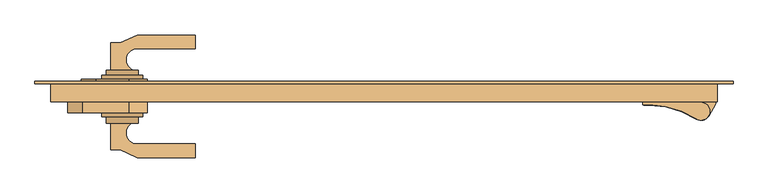
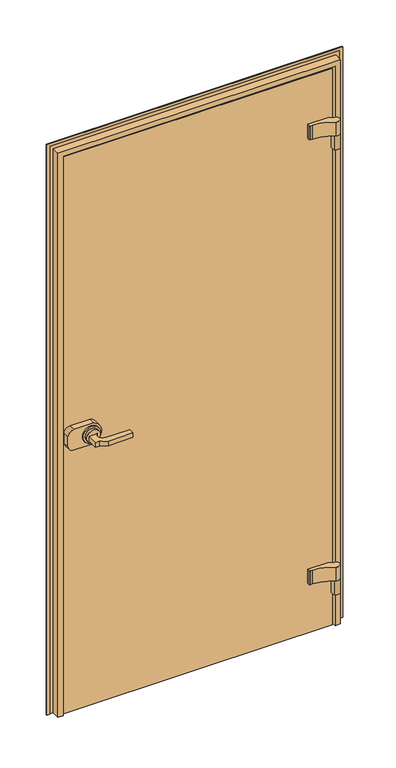
"""IFC4 building model written with IfcOpenShell, lengths in millimetres: door geometry, Doors_Doors_Faraone_Anta : Doors_Doors_Faraone_Anta."""

from ifc_helpers import new_model, si_unit, point, frame, frame_2d, origin, place, context, project, spatial, polyline, circle_curve, trimmed, segment, composite_curve, outline, extrude, faceted_brep, source, transform, mapped, element, save


def door_472ffe8c(model_context):
    return source(origin(), model_context, "Body", "SolidModel", [
        extrude(outline(polyline([(376.5509112, 11.599726), (446.250386, 11.599726), (446.250386, 1.8997991), (376.5509112, 1.8997991), (376.5509112, 11.599726)])), frame((0.0, 0.0, 1799.0000277), z_axis=(0.0, 0.0, 1.0), x_axis=(1.0, 0.0, 0.0)), (0.0, 0.0, 1.0), 50.0),
        extrude(outline(composite_curve([segment(polyline([(376.5509112, -17.600054), (376.5509112, -8.1001256), (446.5503838, -8.1001256), (446.5503838, -9.6001143), (466.1896331, -16.9560894)]), True, "CONTINUOUS"), segment(trimmed(circle_curve(frame_2d((461.5502708, -29.0999673)), 12.9999021), [point((466.1896331, -16.9560894))], [point((454.7624862, -40.1870515))], False, "CARTESIAN"), True, "CONTINUOUS"), segment(trimmed(circle_curve(frame_2d((385.1363002, -147.5843675)), 127.9921454), [point((454.7624862, -40.1870515))], [point((386.5508359, -19.6000389))], True, "CARTESIAN"), True, "CONTINUOUS"), segment(polyline([(386.5508359, -19.6000389), (378.5508961, -19.6000389)]), True, "CONTINUOUS"), segment(trimmed(circle_curve(frame_2d((378.5508961, -17.600054)), 1.9999849), [point((378.5508961, -19.6000389))], [point((376.5509112, -17.600054))], False, "CARTESIAN"), True, "CONTINUOUS")], self_intersect=False)), frame((0.0, 0.0, 1799.0000277), z_axis=(0.0, 0.0, 1.0), x_axis=(1.0, 0.0, 0.0)), (0.0, 0.0, 1.0), 50.0),
        extrude(outline(composite_curve([segment(polyline([(483.3501065, -18.0609582), (472.573012, -35.9917471)]), True, "CONTINUOUS"), segment(trimmed(circle_curve(frame_2d((461.5502708, -29.0999673)), 12.9999021), [point((472.573012, -35.9917471))], [point((451.2009633, -36.9669419))], False, "CARTESIAN"), True, "CONTINUOUS"), segment(trimmed(circle_curve(frame_2d((461.5502708, -29.0999673)), 12.9999021), [point((451.2009633, -36.9669419))], [point((457.1671339, -16.861276))], False, "CARTESIAN"), True, "CONTINUOUS"), segment(polyline([(457.1671339, -16.861276), (461.5537493, -15.0000736), (483.3501065, -15.0000736), (483.3501065, -18.0609582)]), True, "CONTINUOUS")], self_intersect=False)), frame((0.0, 0.0, 1749.0000277), z_axis=(0.0, 0.0, 1.0), x_axis=(1.0, 0.0, 0.0)), (0.0, 0.0, 1.0), 50.0),
        extrude(outline(polyline([(376.5509112, 11.599726), (446.250386, 11.599726), (446.250386, 1.8997991), (376.5509112, 1.8997991), (376.5509112, 11.599726)])), frame((0.0, 0.0, 182.0), z_axis=(0.0, 0.0, 1.0), x_axis=(1.0, 0.0, 0.0)), (0.0, 0.0, 1.0), 50.0),
        extrude(outline(composite_curve([segment(polyline([(376.5509112, -17.600054), (376.5509112, -8.1001256), (446.5503838, -8.1001256), (446.5503838, -9.6001143), (466.1896331, -16.9560894)]), True, "CONTINUOUS"), segment(trimmed(circle_curve(frame_2d((461.5502708, -29.0999673)), 12.9999021), [point((466.1896331, -16.9560894))], [point((454.7624862, -40.1870515))], False, "CARTESIAN"), True, "CONTINUOUS"), segment(trimmed(circle_curve(frame_2d((385.1363002, -147.5843675)), 127.9921454), [point((454.7624862, -40.1870515))], [point((386.5508359, -19.6000389))], True, "CARTESIAN"), True, "CONTINUOUS"), segment(polyline([(386.5508359, -19.6000389), (378.5508961, -19.6000389)]), True, "CONTINUOUS"), segment(trimmed(circle_curve(frame_2d((378.5508961, -17.600054)), 1.9999849), [point((378.5508961, -19.6000389))], [point((376.5509112, -17.600054))], False, "CARTESIAN"), True, "CONTINUOUS")], self_intersect=False)), frame((0.0, 0.0, 182.0), z_axis=(0.0, 0.0, 1.0), x_axis=(1.0, 0.0, 0.0)), (0.0, 0.0, 1.0), 50.0),
        extrude(outline(composite_curve([segment(polyline([(483.3501065, -18.0609582), (472.573012, -35.9917471)]), True, "CONTINUOUS"), segment(trimmed(circle_curve(frame_2d((461.5502708, -29.0999673)), 12.9999021), [point((472.573012, -35.9917471))], [point((451.2009633, -36.9669419))], False, "CARTESIAN"), True, "CONTINUOUS"), segment(trimmed(circle_curve(frame_2d((461.5502708, -29.0999673)), 12.9999021), [point((451.2009633, -36.9669419))], [point((457.1671339, -16.861276))], False, "CARTESIAN"), True, "CONTINUOUS"), segment(polyline([(457.1671339, -16.861276), (461.5537493, -15.0000736), (483.3501065, -15.0000736), (483.3501065, -18.0609582)]), True, "CONTINUOUS")], self_intersect=False)), frame((0.0, 0.0, 132.0), z_axis=(0.0, 0.0, 1.0), x_axis=(1.0, 0.0, 0.0)), (0.0, 0.0, 1.0), 50.0),
        extrude(outline(composite_curve([segment(trimmed(circle_curve(frame_2d((1003.2884985, -381.2459675)), 23.0897305), [point((1003.2884985, -404.335698))], [point((1003.2884985, -358.156237))], False, "CARTESIAN"), True, "CONTINUOUS"), segment(trimmed(circle_curve(frame_2d((1003.2884985, -381.2459675)), 23.0897305), [point((1003.2884985, -358.156237))], [point((1003.2884985, -404.335698))], False, "CARTESIAN"), True, "CONTINUOUS")], self_intersect=False)), frame((0.0, -46.355004, 0.0), z_axis=(0.0, 1.0, 0.0), x_axis=(0.0, 0.0, 1.0)), (0.0, 0.0, 1.0), 9.3686894),
        extrude(outline(composite_curve([segment(trimmed(circle_curve(frame_2d((987.7717852, -438.83347)), 22.4105262), [point((983.5880679, -460.8500137))], [point((965.361259, -438.83347))], False, "CARTESIAN"), True, "CONTINUOUS"), segment(polyline([(965.361259, -438.83347), (965.361259, -373.83347)]), True, "CONTINUOUS"), segment(trimmed(circle_curve(frame_2d((1002.861259, -383.4990023)), 38.7256054), [point((965.361259, -373.83347))], [point((1039.5100566, -370.9874819))], False, "CARTESIAN"), True, "CONTINUOUS"), segment(polyline([(1039.5100566, -370.9874819), (1039.5100566, -438.83347)]), True, "CONTINUOUS"), segment(trimmed(circle_curve(frame_2d((1017.0995304, -438.83347)), 22.4105262), [point((1039.5100566, -438.83347))], [point((1021.2832478, -460.8500137))], False, "CARTESIAN"), True, "CONTINUOUS"), segment(polyline([(1021.2832478, -460.8500137), (983.5880679, -460.8500137)]), True, "CONTINUOUS")], self_intersect=False)), frame((0.0, -31.1653283, 0.0), z_axis=(0.0, 1.0, 0.0), x_axis=(0.0, 0.0, 1.0)), (0.0, 0.0, 1.0), 23.0652027),
        extrude(outline(composite_curve([segment(trimmed(circle_curve(frame_2d((987.7717852, -438.83347)), 22.4105262), [point((983.5880679, -460.8500137))], [point((965.361259, -438.83347))], False, "CARTESIAN"), True, "CONTINUOUS"), segment(polyline([(965.361259, -438.83347), (965.361259, -373.83347)]), True, "CONTINUOUS"), segment(trimmed(circle_curve(frame_2d((1002.861259, -383.4990023)), 38.7256054), [point((965.361259, -373.83347))], [point((1039.5100566, -370.9874819))], False, "CARTESIAN"), True, "CONTINUOUS"), segment(polyline([(1039.5100566, -370.9874819), (1039.5100566, -438.83347)]), True, "CONTINUOUS"), segment(trimmed(circle_curve(frame_2d((1017.0995304, -438.83347)), 22.4105262), [point((1039.5100566, -438.83347))], [point((1021.2832478, -460.8500137))], False, "CARTESIAN"), True, "CONTINUOUS"), segment(polyline([(1021.2832478, -460.8500137), (983.5880679, -460.8500137)]), True, "CONTINUOUS")], self_intersect=False)), frame((0.0, -31.1653283, 0.0), z_axis=(0.0, 1.0, 0.0), x_axis=(0.0, 0.0, 1.0)), (0.0, 0.0, 1.0), 23.0652027),
        extrude(outline(composite_curve([segment(trimmed(circle_curve(frame_2d((1003.2884985, -381.2459675)), 30.0), [point((1003.2884985, -411.2459675))], [point((1003.2884985, -351.2459675))], False, "CARTESIAN"), True, "CONTINUOUS"), segment(trimmed(circle_curve(frame_2d((1003.2884985, -381.2459675)), 30.0), [point((1003.2884985, -351.2459675))], [point((1003.2884985, -411.2459675))], False, "CARTESIAN"), True, "CONTINUOUS")], self_intersect=False)), frame((0.0, -36.9863146, 0.0), z_axis=(0.0, 1.0, 0.0), x_axis=(0.0, 0.0, 1.0)), (0.0, 0.0, 1.0), 5.8209863),
        extrude(outline(composite_curve([segment(trimmed(circle_curve(frame_2d((987.7717852, -438.83347)), 22.4105262), [point((983.5880679, -460.8500137))], [point((965.361259, -438.83347))], False, "CARTESIAN"), True, "CONTINUOUS"), segment(polyline([(965.361259, -438.83347), (965.361259, -373.83347)]), True, "CONTINUOUS"), segment(trimmed(circle_curve(frame_2d((1002.861259, -383.4990023)), 38.7256054), [point((965.361259, -373.83347))], [point((1039.5100566, -370.9874819))], False, "CARTESIAN"), True, "CONTINUOUS"), segment(polyline([(1039.5100566, -370.9874819), (1039.5100566, -438.83347)]), True, "CONTINUOUS"), segment(trimmed(circle_curve(frame_2d((1017.0995304, -438.83347)), 22.4105262), [point((1039.5100566, -438.83347))], [point((1021.2832478, -460.8500137))], False, "CARTESIAN"), True, "CONTINUOUS"), segment(polyline([(1021.2832478, -460.8500137), (983.5880679, -460.8500137)]), True, "CONTINUOUS")], self_intersect=False)), frame((0.0, -31.1653283, 0.0), z_axis=(0.0, 1.0, 0.0), x_axis=(0.0, 0.0, 1.0)), (0.0, 0.0, 1.0), 23.0652027),
        extrude(outline(composite_curve([segment(trimmed(circle_curve(frame_2d((1003.2884985, -381.2459675)), 23.0897305), [point((1003.2884985, -404.335698))], [point((1003.2884985, -358.156237))], False, "CARTESIAN"), True, "CONTINUOUS"), segment(trimmed(circle_curve(frame_2d((1003.2884985, -381.2459675)), 23.0897305), [point((1003.2884985, -358.156237))], [point((1003.2884985, -404.335698))], False, "CARTESIAN"), True, "CONTINUOUS")], self_intersect=False)), frame((0.0, -46.355004, 0.0), z_axis=(0.0, 1.0, 0.0), x_axis=(0.0, 0.0, 1.0)), (0.0, 0.0, 1.0), 14.1896757),
        extrude(outline(composite_curve([segment(trimmed(circle_curve(frame_2d((987.7717852, -438.83347)), 22.4105262), [point((983.5880679, -460.8500137))], [point((965.361259, -438.83347))], False, "CARTESIAN"), True, "CONTINUOUS"), segment(polyline([(965.361259, -438.83347), (965.361259, -373.83347)]), True, "CONTINUOUS"), segment(trimmed(circle_curve(frame_2d((1002.861259, -383.4990023)), 38.7256054), [point((965.361259, -373.83347))], [point((1039.5100566, -370.9874819))], False, "CARTESIAN"), True, "CONTINUOUS"), segment(polyline([(1039.5100566, -370.9874819), (1039.5100566, -438.83347)]), True, "CONTINUOUS"), segment(trimmed(circle_curve(frame_2d((1017.0995304, -438.83347)), 22.4105262), [point((1039.5100566, -438.83347))], [point((1021.2832478, -460.8500137))], False, "CARTESIAN"), True, "CONTINUOUS"), segment(polyline([(1021.2832478, -460.8500137), (983.5880679, -460.8500137)]), True, "CONTINUOUS")], self_intersect=False)), frame((0.0, -31.1653283, 0.0), z_axis=(0.0, 1.0, 0.0), x_axis=(0.0, 0.0, 1.0)), (0.0, 0.0, 1.0), 23.0652027),
        extrude(outline(composite_curve([segment(trimmed(circle_curve(frame_2d((987.7717852, -438.83347)), 22.4105262), [point((983.5880679, -460.8500137))], [point((965.361259, -438.83347))], False, "CARTESIAN"), True, "CONTINUOUS"), segment(polyline([(965.361259, -438.83347), (965.361259, -373.83347)]), True, "CONTINUOUS"), segment(trimmed(circle_curve(frame_2d((1002.861259, -383.4990023)), 38.7256054), [point((965.361259, -373.83347))], [point((1039.5100566, -370.9874819))], False, "CARTESIAN"), True, "CONTINUOUS"), segment(polyline([(1039.5100566, -370.9874819), (1039.5100566, -438.83347)]), True, "CONTINUOUS"), segment(trimmed(circle_curve(frame_2d((1017.0995304, -438.83347)), 22.4105262), [point((1039.5100566, -438.83347))], [point((1021.2832478, -460.8500137))], False, "CARTESIAN"), True, "CONTINUOUS"), segment(polyline([(1021.2832478, -460.8500137), (983.5880679, -460.8500137)]), True, "CONTINUOUS")], self_intersect=False)), frame((0.0, -31.1653283, 0.0), z_axis=(0.0, 1.0, 0.0), x_axis=(0.0, 0.0, 1.0)), (0.0, 0.0, 1.0), 23.0652027),
        extrude(outline(composite_curve([segment(polyline([(-397.6805645, -84.9663543), (-397.6805645, -46.355004), (-367.7217579, -46.355004)]), True, "CONTINUOUS"), segment(trimmed(circle_curve(frame_2d((-359.5544088, -60.2485058)), 16.1162956), [point((-367.7217579, -46.355004))], [point((-359.5544088, -76.3648014))], True, "CARTESIAN"), True, "CONTINUOUS"), segment(polyline([(-359.5544088, -76.3648014), (-274.5544088, -76.3648014), (-274.5544088, -96.3648014), (-359.5544088, -96.3648014), (-383.9984574, -84.9663543), (-397.6805645, -84.9663543)]), True, "CONTINUOUS")], self_intersect=False)), frame((0.0, 0.0, 992.5658854), z_axis=(0.0, 0.0, 1.0), x_axis=(1.0, 0.0, 0.0)), (0.0, 0.0, 1.0), 16.6938628),
        extrude(outline(composite_curve([segment(trimmed(circle_curve(frame_2d((987.7717852, -438.83347)), 22.4105262), [point((983.5880679, -460.8500137))], [point((965.361259, -438.83347))], False, "CARTESIAN"), True, "CONTINUOUS"), segment(polyline([(965.361259, -438.83347), (965.361259, -373.83347)]), True, "CONTINUOUS"), segment(trimmed(circle_curve(frame_2d((1002.861259, -383.4990023)), 38.7256054), [point((965.361259, -373.83347))], [point((1039.5100566, -370.9874819))], False, "CARTESIAN"), True, "CONTINUOUS"), segment(polyline([(1039.5100566, -370.9874819), (1039.5100566, -438.83347)]), True, "CONTINUOUS"), segment(trimmed(circle_curve(frame_2d((1017.0995304, -438.83347)), 22.4105262), [point((1039.5100566, -438.83347))], [point((1021.2832478, -460.8500137))], False, "CARTESIAN"), True, "CONTINUOUS"), segment(polyline([(1021.2832478, -460.8500137), (983.5880679, -460.8500137)]), True, "CONTINUOUS")], self_intersect=False)), frame((0.0, -31.1653283, 0.0), z_axis=(0.0, 1.0, 0.0), x_axis=(0.0, 0.0, 1.0)), (0.0, 0.0, 1.0), 23.0652027),
        extrude(outline(composite_curve([segment(trimmed(circle_curve(frame_2d((1003.2884985, -381.2459675)), 23.0897305), [point((1003.2884985, -404.335698))], [point((1003.2884985, -358.156237))], False, "CARTESIAN"), True, "CONTINUOUS"), segment(trimmed(circle_curve(frame_2d((1003.2884985, -381.2459675)), 23.0897305), [point((1003.2884985, -358.156237))], [point((1003.2884985, -404.335698))], False, "CARTESIAN"), True, "CONTINUOUS")], self_intersect=False)), frame((0.0, 23.8998744, 0.0), z_axis=(0.0, 1.0, 0.0), x_axis=(0.0, 0.0, 1.0)), (0.0, 0.0, 1.0), 7.0),
        extrude(outline(composite_curve([segment(trimmed(circle_curve(frame_2d((987.7717852, -418.83347)), 22.4105262), [point((983.5880679, -440.8500137))], [point((965.361259, -418.83347))], False, "CARTESIAN"), True, "CONTINUOUS"), segment(polyline([(965.361259, -418.83347), (965.361259, -373.83347)]), True, "CONTINUOUS"), segment(trimmed(circle_curve(frame_2d((1002.861259, -383.4990023)), 38.7256054), [point((965.361259, -373.83347))], [point((1039.5100566, -370.9874819))], False, "CARTESIAN"), True, "CONTINUOUS"), segment(polyline([(1039.5100566, -370.9874819), (1039.5100566, -418.83347)]), True, "CONTINUOUS"), segment(trimmed(circle_curve(frame_2d((1017.0995304, -418.83347)), 22.4105262), [point((1039.5100566, -418.83347))], [point((1021.2832478, -440.8500137))], False, "CARTESIAN"), True, "CONTINUOUS"), segment(polyline([(1021.2832478, -440.8500137), (983.5880679, -440.8500137)]), True, "CONTINUOUS")], self_intersect=False)), frame((0.0, 1.8998744, 0.0), z_axis=(0.0, 1.0, 0.0), x_axis=(0.0, 0.0, 1.0)), (0.0, 0.0, 1.0), 16.0),
        extrude(outline(composite_curve([segment(polyline([(-397.6805645, 70.762087), (-383.9984574, 70.762087), (-359.5544088, 82.1605341), (-274.5544088, 82.1605341), (-274.5544088, 62.1605341), (-359.5544088, 62.1605341)]), True, "CONTINUOUS"), segment(trimmed(circle_curve(frame_2d((-359.5544088, 46.0442385)), 16.1162956), [point((-359.5544088, 62.1605341))], [point((-365.0665065, 30.8998744))], True, "CARTESIAN"), True, "CONTINUOUS"), segment(polyline([(-365.0665065, 30.8998744), (-397.6805645, 30.8998744), (-397.6805645, 70.762087)]), True, "CONTINUOUS")], self_intersect=False)), frame((0.0, 0.0, 992.5658854), z_axis=(0.0, 0.0, 1.0), x_axis=(1.0, 0.0, 0.0)), (0.0, 0.0, 1.0), 16.6938628),
        extrude(outline(composite_curve([segment(trimmed(circle_curve(frame_2d((1003.2884985, -381.2459675)), 30.0), [point((1003.2884985, -411.2459675))], [point((1003.2884985, -351.2459675))], False, "CARTESIAN"), True, "CONTINUOUS"), segment(trimmed(circle_curve(frame_2d((1003.2884985, -381.2459675)), 30.0), [point((1003.2884985, -351.2459675))], [point((1003.2884985, -411.2459675))], False, "CARTESIAN"), True, "CONTINUOUS")], self_intersect=False)), frame((0.0, 17.8998744, 0.0), z_axis=(0.0, 1.0, 0.0), x_axis=(0.0, 0.0, 1.0)), (0.0, 0.0, 1.0), 6.0),
        faceted_brep([(-452.3502762, 14.999774, 0.0), (-452.3502762, 5.9998078, 0.0), (-467.3501757, 5.9998078, 0.0), (-467.3501757, -15.0, 0.0), (-485.3500137, -15.0, 0.0), (-485.3500137, 12.9997254, 0.0), (-499.0499489, 12.9997254, 0.0), (-499.0499489, 11.2997382, 0.0), (-508.3498379, 11.2997382, 0.0), (-508.3498379, 14.999774, 0.0), (-452.3502762, 14.999774, 2017.0002901), (-452.3502762, 5.9998078, 2017.0002901), (452.3502762, 5.9998078, 2017.0002901), (452.3502762, 5.9998078, 0.0), (467.3501757, 5.9998078, 0.0), (467.3501757, 5.9998078, 2032.0001896), (-467.3501757, 5.9998078, 2032.0001896), (-467.3501757, -15.0, 2032.0001896), (467.3501757, -15.0, 2032.0001896), (467.3501757, -15.0, 0.0), (485.3500137, -15.0, 0.0), (485.3500137, -15.0, 2050.0000277), (-485.3500137, -15.0, 2050.0000277), (-485.3500137, 12.9997254, 2050.0000277), (485.3500137, 12.9997254, 2050.0000277), (485.3500137, 12.9997254, 0.0), (499.0499489, 12.9997254, 0.0), (499.0499489, 12.9997254, 2063.6999629), (-499.0499489, 12.9997254, 2063.6999629), (-499.0499489, 11.2997382, 2063.6999629), (499.0499489, 11.2997382, 2063.6999629), (499.0499489, 11.2997382, 0.0), (508.3498379, 11.2997382, 0.0), (508.3498379, 11.2997382, 2072.9998518), (-508.3498379, 11.2997382, 2072.9998518), (-508.3498379, 14.999774, 2072.9998518), (508.3498379, 14.999774, 2072.9998518), (508.3498379, 14.999774, 0.0), (452.3502762, 14.999774, 0.0), (452.3502762, 14.999774, 2017.0002901)], [[[0, 1, 2, 3, 4, 5, 6, 7, 8, 9]], [[1, 0, 10, 11]], [[2, 1, 11, 12, 13, 14, 15, 16]], [[3, 2, 16, 17]], [[4, 3, 17, 18, 19, 20, 21, 22]], [[5, 4, 22, 23]], [[6, 5, 23, 24, 25, 26, 27, 28]], [[7, 6, 28, 29]], [[8, 7, 29, 30, 31, 32, 33, 34]], [[9, 8, 34, 35]], [[0, 9, 35, 36, 37, 38, 39, 10]], [[12, 39, 38, 13]], [[38, 37, 32, 31, 26, 25, 20, 19, 14, 13]], [[18, 15, 14, 19]], [[24, 21, 20, 25]], [[30, 27, 26, 31]], [[36, 33, 32, 37]], [[11, 10, 39, 12]], [[17, 16, 15, 18]], [[23, 22, 21, 24]], [[29, 28, 27, 30]], [[35, 34, 33, 36]]]),
        extrude(outline(polyline([(0.0, -460.8500137), (0.0, 9.5), (0.0, 460.8500137), (2023.9998511, 460.8500137), (2023.9998511, -460.8500137), (0.0, -460.8500137)])), frame((0.0, -8.1001256, 0.0), z_axis=(0.0, 1.0, 0.0), x_axis=(0.0, 0.0, 1.0)), (0.0, 0.0, 1.0), 10.0),
    ])


if __name__ == "__main__":
    model = new_model("IFC4")
    model_context = context("Model", 3, world=origin())
    ifc_project = project(units=[si_unit("LENGTHUNIT", "METRE", prefix="MILLI")], contexts=[model_context])
    site = spatial("IfcSite", under=ifc_project)
    building = spatial("IfcBuilding", under=site)
    placement = place(None, origin())
    door_shape = door_472ffe8c(model_context)
    element("IfcDoor", 1, ObjectType="Doors_Doors_Faraone_Anta : Doors_Doors_Faraone_Anta", at=placement, inside=building, context=model_context, shape_type="MappedRepresentation", body=[
        mapped(door_shape, transform((0.0, 0.0, 0.0), x_axis=(1.0, 0.0, 0.0), y_axis=(0.0, 1.0, 0.0), z_axis=(0.0, 0.0, 1.0))),
    ])
    save(model, "model.ifc")

# Revit data of these elements
# Type "Doors_Doors_Faraone_Anta : Doors_Doors_Faraone_Anta"
#   Type Mark = "58"
#   URL = "https://faraone.it/en/"
#   Product data url = ""
#   Product Guid = ""
#   Model = "Spazio_Anta"
#   Manufacturer = "Faraone"
#   Keynote = "08110"
#   Assembly Code = "C1020100"
#   Analytic Construction = "<None>"
#   Width [instance default] = 1104.999 mm
#   Height [instance default] = 2700 mm
#   Handle Height = 1000 mm
#   Thickness = 11 mm
#   Glass Width [instance default] = 1055.999 mm
#   Middle Hinge [instance default] = yes
#   Edition number = 1
#   Define Thermal Properties by = 1
#   Interior Material = Glass - Faraone - Transparent
#   Handle Type = element 507032
#   Exterior Material = Aluminium - Faraone - Silver
#   Function = (empty or 0)
# Element 1 (IfcDoor, "Doors_Doors_Faraone_Anta : Doors_Doors_Faraone_Anta")
#   Width = 970.7 mm
#   Height = 2050 mm
#   Glass Width = 921.7 mm
#   Middle Hinge = no
#   Materials on its faces: "Aluminium - Faraone - Silver", "Glass - Faraone - Transparent"
# Materials
#   "Glass - Faraone - Transparent": class "Glass", colour RGB 0 128 192, transparency 0.9, Description = "Soda Lime Glass", Cost = 0
#   "Aluminium - Faraone - Silver": class "Metal", colour RGB 244 244 244, transparency 0, Description = "Metal - Faraone - Aluminium", Cost = 0
